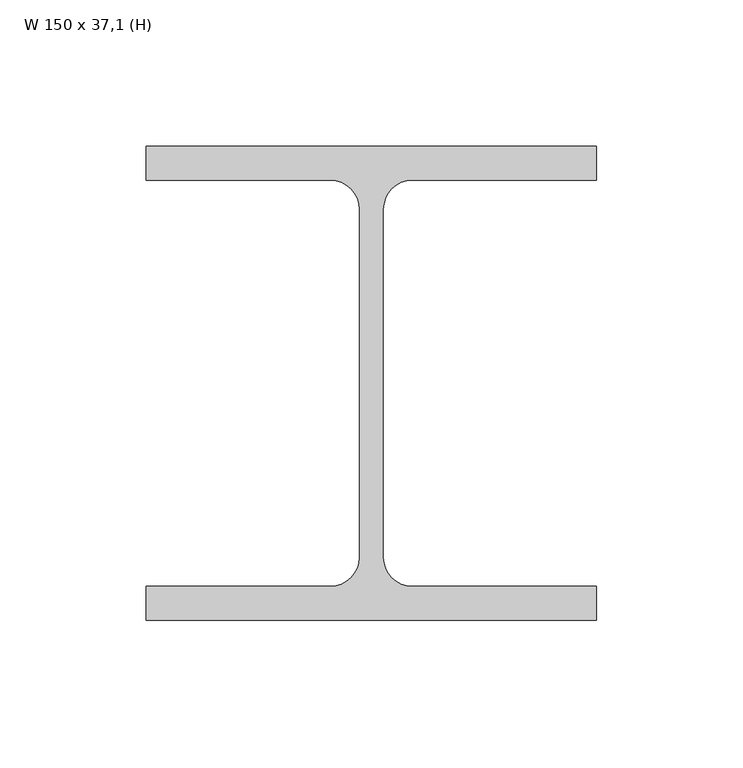
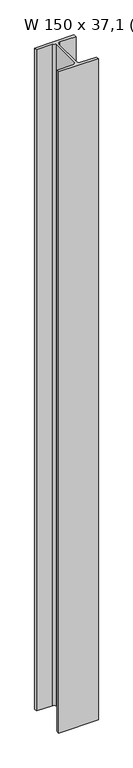
"""IFC4 building model written with IfcOpenShell, lengths in millimetres: column geometry, Pilar de Aço - H : W 150 x 37,1 (H)."""

from ifc_helpers import new_model, si_unit, point, frame_2d, origin, origin_with_axes, place, context, project, spatial, polyline, circle_curve, trimmed, segment, composite_curve, outline, extrude, source, transform, mapped, element, save


def w_150_x_37_1_h_ba3580ec(model_context):
    return source(origin(), model_context, "Body", "SweptSolid", [
        extrude(outline(composite_curve([segment(polyline([(77.0, 81.0), (77.0, 69.4), (13.95, 69.4)]), True, "CONTINUOUS"), segment(trimmed(circle_curve(frame_2d((13.95, 59.5)), 9.9), [point((13.95, 69.4))], [point((4.05, 59.5))], True, "CARTESIAN"), True, "CONTINUOUS"), segment(polyline([(4.05, 59.5), (4.05, -59.5)]), True, "CONTINUOUS"), segment(trimmed(circle_curve(frame_2d((13.95, -59.5)), 9.9), [point((4.05, -59.5))], [point((13.95, -69.4))], True, "CARTESIAN"), True, "CONTINUOUS"), segment(polyline([(13.95, -69.4), (77.0, -69.4), (77.0, -81.0), (-77.0, -81.0), (-77.0, -69.4), (-13.95, -69.4)]), True, "CONTINUOUS"), segment(trimmed(circle_curve(frame_2d((-13.95, -59.5)), 9.9), [point((-13.95, -69.4))], [point((-4.05, -59.5))], True, "CARTESIAN"), True, "CONTINUOUS"), segment(polyline([(-4.05, -59.5), (-4.05, 59.5)]), True, "CONTINUOUS"), segment(trimmed(circle_curve(frame_2d((-13.95, 59.5)), 9.9), [point((-4.05, 59.5))], [point((-13.95, 69.4))], True, "CARTESIAN"), True, "CONTINUOUS"), segment(polyline([(-13.95, 69.4), (-77.0, 69.4), (-77.0, 81.0), (77.0, 81.0)]), True, "CONTINUOUS")], self_intersect=False)), origin_with_axes(), (0.0, 0.0, 1.0), 2720.0),
    ])


if __name__ == "__main__":
    model = new_model("IFC4")
    model_context = context("Model", 3, world=origin())
    ifc_project = project(units=[si_unit("LENGTHUNIT", "METRE", prefix="MILLI")], contexts=[model_context])
    site = spatial("IfcSite", under=ifc_project)
    building = spatial("IfcBuilding", under=site)
    placement = place(None, origin())
    w_150_x_37_1_h_shape = w_150_x_37_1_h_ba3580ec(model_context)
    element("IfcColumn", 1, ObjectType="Pilar de Aço - H : W 150 x 37,1 (H)", at=placement, inside=building, context=model_context, shape_type="MappedRepresentation", body=[
        mapped(w_150_x_37_1_h_shape, transform((0.0, 0.0, 0.0), x_axis=(1.0, 0.0, 0.0), y_axis=(0.0, 1.0, 0.0), z_axis=(0.0, 0.0, 1.0))),
    ])
    save(model, "model.ifc")

# Revit data of these elements
# Type "Pilar de Aço - H : W 150 x 37,1 (H)"
#   SINAPI = ""
#   Área da seção = 47.8 m²
#   tw = 0.81 cm
#   tf = 1.16 cm
#   h = 13.88 cm
#   d' = 11.90 cm
#   d = 16.20 cm
#   bf = 15.40 cm
#   R = 0.99 cm
#   Massa Linear kg/m = 37.1
#   Aço = Metal - Aço 345MPa
#   Assembly Code = ""
# Materials
#   "Metal - Aço 345MPa": class "Metal", colour RGB 189 187 185, transparency 0, Cost = 0
